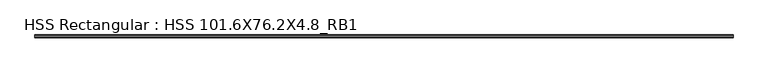
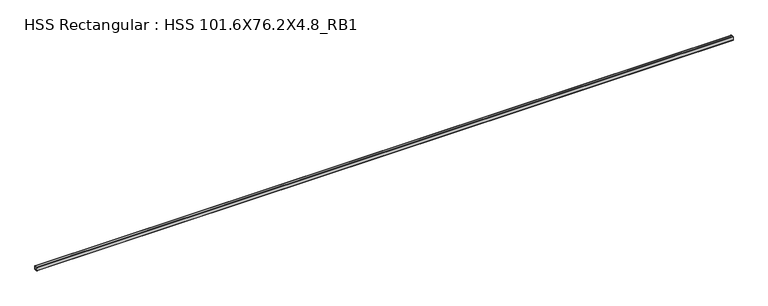
"""IFC4 building model written with IfcOpenShell, lengths in millimetres: beam geometry, HSS Rectangular : HSS 101.6X76.2X4.8_RB1."""

from ifc_helpers import new_model, si_unit, point, frame, frame_2d, origin, place, context, project, spatial, polyline, circle_curve, trimmed, segment, composite_curve, outline, extrude, source, transform, mapped, element, save


def hss_rectangular_hss_101_6x76_2x4_8_rb1_308b899f(model_context):
    return source(origin(), model_context, "Body", "SweptSolid", [
        extrude(outline(composite_curve([segment(trimmed(circle_curve(frame_2d((-28.575, 41.275)), 9.525), [point((-38.1, 41.275))], [point((-28.575, 50.8))], False, "CARTESIAN"), True, "CONTINUOUS"), segment(polyline([(-28.575, 50.8), (28.575, 50.8)]), True, "CONTINUOUS"), segment(trimmed(circle_curve(frame_2d((28.575, 41.275)), 9.525), [point((28.575, 50.8))], [point((38.1, 41.275))], False, "CARTESIAN"), True, "CONTINUOUS"), segment(polyline([(38.1, 41.275), (38.1, -41.275)]), True, "CONTINUOUS"), segment(trimmed(circle_curve(frame_2d((28.575, -41.275)), 9.525), [point((38.1, -41.275))], [point((28.575, -50.8))], False, "CARTESIAN"), True, "CONTINUOUS"), segment(polyline([(28.575, -50.8), (-28.575, -50.8)]), True, "CONTINUOUS"), segment(trimmed(circle_curve(frame_2d((-28.575, -41.275)), 9.525), [point((-28.575, -50.8))], [point((-38.1, -41.275))], False, "CARTESIAN"), True, "CONTINUOUS"), segment(polyline([(-38.1, -41.275), (-38.1, 41.275)]), True, "CONTINUOUS")], self_intersect=False), holes=[composite_curve([segment(polyline([(28.575, 46.0375), (-28.575, 46.0375)]), True, "CONTINUOUS"), segment(trimmed(circle_curve(frame_2d((-28.575, 41.275)), 4.7625), [point((-28.575, 46.0375))], [point((-33.3375, 41.275))], True, "CARTESIAN"), True, "CONTINUOUS"), segment(polyline([(-33.3375, 41.275), (-33.3375, -41.275)]), True, "CONTINUOUS"), segment(trimmed(circle_curve(frame_2d((-28.575, -41.275)), 4.7625), [point((-33.3375, -41.275))], [point((-28.575, -46.0375))], True, "CARTESIAN"), True, "CONTINUOUS"), segment(polyline([(-28.575, -46.0375), (28.575, -46.0375)]), True, "CONTINUOUS"), segment(trimmed(circle_curve(frame_2d((28.575, -41.275)), 4.7625), [point((28.575, -46.0375))], [point((33.3375, -41.275))], True, "CARTESIAN"), True, "CONTINUOUS"), segment(polyline([(33.3375, -41.275), (33.3375, 41.275)]), True, "CONTINUOUS"), segment(trimmed(circle_curve(frame_2d((28.575, 41.275)), 4.7625), [point((33.3375, 41.275))], [point((28.575, 46.0375))], True, "CARTESIAN"), True, "CONTINUOUS")], self_intersect=False)]), frame((-7490.0, 0.0, 0.0), z_axis=(1.0, 0.0, 0.0), x_axis=(0.0, 1.0, 0.0)), (0.0, 0.0, 1.0), 18018.4315897),
    ])


if __name__ == "__main__":
    model = new_model("IFC4")
    model_context = context("Model", 3, world=origin())
    ifc_project = project(units=[si_unit("LENGTHUNIT", "METRE", prefix="MILLI")], contexts=[model_context])
    site = spatial("IfcSite", under=ifc_project)
    building = spatial("IfcBuilding", under=site)
    placement = place(None, origin())
    hss_rectangular_hss_101_6x76_2x4_8_rb1_shape = hss_rectangular_hss_101_6x76_2x4_8_rb1_308b899f(model_context)
    element("IfcBeam", 1, ObjectType="HSS Rectangular : HSS 101.6X76.2X4.8_RB1", at=placement, inside=building, context=model_context, shape_type="MappedRepresentation", body=[
        mapped(hss_rectangular_hss_101_6x76_2x4_8_rb1_shape, transform((0.0, 0.0, 0.0), x_axis=(1.0, 0.0, 0.0), y_axis=(0.0, 1.0, 0.0), z_axis=(0.0, 0.0, 1.0))),
    ])
    save(model, "model.ifc")

# Revit data of these elements
# Type "HSS Rectangular : HSS 101.6X76.2X4.8_RB1"
#   Section Name Key = "HSS 4X3X3/16"
#   Assembly Code = "B10"
#   Width = 7.62 cm
#   Wall Nominal Thickness = 0.4763 cm
#   Wall Design Thickness = 0.442 cm
#   Torsional Moment of Inertia = 260.561 cm⁴
#   Torsional Modulus = 61.2876 cm³
#   Section Area = 14.4516 cm²
#   Plastic Modulus weak axis = 40.3122 cm³
#   Plastic Modulus strong axis = 49.1612 cm³
#   Perimeter = 0.881482 m²/m
#   Outer Fillet = 0.9525 cm
#   Nominal Weight = 12.1285 kgf/m
#   Moment of Inertia weak axis = 131.529 cm⁴
#   Moment of Inertia strong axis = 205.202 cm⁴
#   Inner Fillet = 0.4763 cm
#   Height = 10.16 cm
#   Elastic Modulus weak axis = 34.4128 cm³
#   Elastic Modulus strong axis = 40.476 cm³
#   Centroid Vertical = 5.08 cm
#   Centroid Horizontal = 3.81 cm
#   Length [instance default] = 1524 mm
#   Structural Material [instance default] = Steel ASTM A500, Grade B, Rectangular and Square
#   Principal Axes Angle = 0
# Element 1 (IfcBeam, "HSS Rectangular : HSS 101.6X76.2X4.8_RB1")
#   Structural Material = Steel ASTM A992
#   Materials on its faces: "Steel ASTM A992"
# Materials
#   "Steel ASTM A500, Grade B, Rectangular and Square": class "Metal", colour RGB 199 199 199, transparency 0, Description = "Carbon steel", Cost = 0
#   "Steel ASTM A992": class "Metal", colour RGB 199 199 199, transparency 0, Description = "Structural steel 50ksi", Cost = 0
